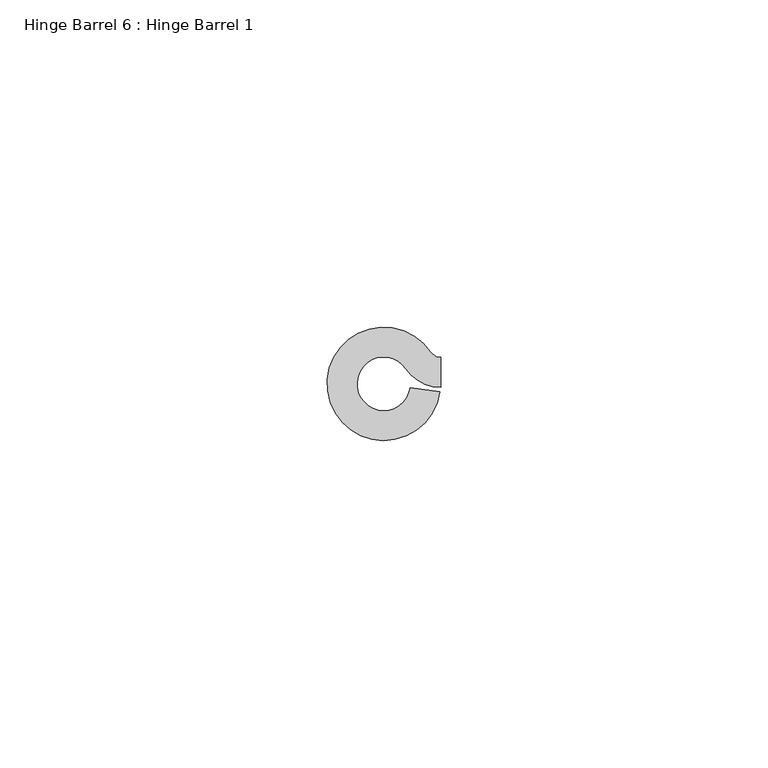
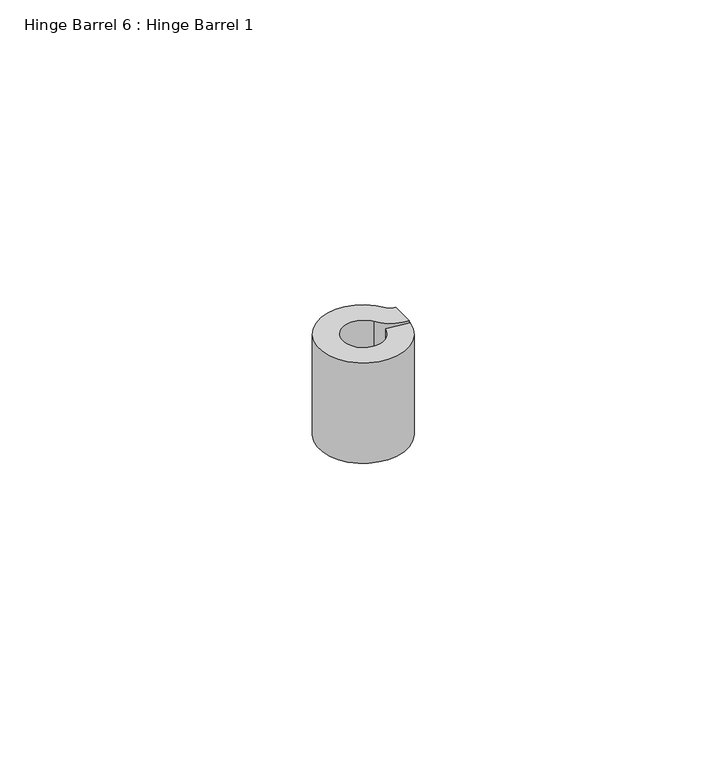
"""IFC4 building model written with IfcOpenShell, lengths in millimetres: proxy geometry, Hinge Barrel 6 : Hinge Barrel 1."""

import ifcopenshell
import ifcopenshell.guid

model = None  # the IFC model being written
_history = None  # IfcOwnerHistory: only IFC2X3 demands one
_inside = {}  # id of a spatial element -> (the spatial element, [elements in it])
_under = {}  # id of a project, library or spatial element -> (it, [spatial elements below it])
_declared = {}  # id of a project -> (the project, [libraries it declares])
_typed = {}  # id of a type object -> (the type object, [elements of that type])
_made_of = {}  # id of a material, layer set ... -> (it, [elements and type objects made of it])


def new_model(schema):
    """Start an empty IFC model of exactly this schema.

    Asked for "IFC4X3", IfcOpenShell would pick the latest addendum, in which some entities
    have other attributes; the version numbers below select the first issue.
    IFC2X3 requires an IfcOwnerHistory on every rooted entity: one is made here for all.
    """
    global model, _history
    if schema == "IFC4X3":
        model = ifcopenshell.file(schema_version=(4, 3, 0, 0))
    else:
        model = ifcopenshell.file(schema=schema)
    _inside.clear()
    _under.clear()
    _declared.clear()
    _typed.clear()
    _made_of.clear()
    _history = None
    if model.schema == "IFC2X3":
        org = make("IfcOrganization", Name="unknown")
        user = make(
            "IfcPersonAndOrganization",
            ThePerson=make("IfcPerson", FamilyName="unknown"),
            TheOrganization=org,
        )
        app = make(
            "IfcApplication",
            ApplicationDeveloper=org,
            Version="unknown",
            ApplicationFullName="unknown",
            ApplicationIdentifier="unknown",
        )
        _history = make(
            "IfcOwnerHistory",
            OwningUser=user,
            OwningApplication=app,
            ChangeAction="ADDED",
            CreationDate=0,
        )
    return model


def make(cls, **values):
    """One entity of the class cls with the attributes given. An attribute that is None is left unset."""
    return model.create_entity(
        cls, **{name: value for name, value in values.items() if value is not None}
    )


def rooted(cls, **values):
    """An entity with a GlobalId (a new one), such as an element, a storey or a relation."""
    return make(cls, GlobalId=ifcopenshell.guid.new(), OwnerHistory=_history, **values)


def si_unit(unit_type, name, prefix=None):
    """IfcSIUnit, for example si_unit("LENGTHUNIT", "METRE", prefix="MILLI")."""
    return make("IfcSIUnit", UnitType=unit_type, Prefix=prefix, Name=name)


def assignment(units):
    """IfcUnitAssignment: the units of a project."""
    return None if units is None else make("IfcUnitAssignment", Units=units)


def point(xyz):
    """IfcCartesianPoint."""
    return None if xyz is None else make("IfcCartesianPoint", Coordinates=xyz)


def direction(xyz):
    """IfcDirection."""
    return None if xyz is None else make("IfcDirection", DirectionRatios=xyz)


def frame(location, z_axis=None, x_axis=None):
    """IfcAxis2Placement3D, a coordinate frame: its origin and axes. An axis left out is left unset."""
    return make(
        "IfcAxis2Placement3D",
        Location=point(location),
        Axis=direction(z_axis),
        RefDirection=direction(x_axis),
    )


def frame_2d(location, x_axis=None):
    """IfcAxis2Placement2D, a coordinate frame in the plane: its origin and x axis."""
    return make(
        "IfcAxis2Placement2D", Location=point(location), RefDirection=direction(x_axis)
    )


def origin():
    """The frame at (0, 0, 0) with its axes left unset."""
    return frame((0.0, 0.0, 0.0))


def place(relative_to, where):
    """IfcLocalPlacement: puts the frame where relative to a parent placement (None: the world)."""
    return make(
        "IfcLocalPlacement", PlacementRelTo=relative_to, RelativePlacement=where
    )


def context(
    kind, dimensions, precision=None, world=None, true_north=None, identifier=None
):
    """IfcGeometricRepresentationContext, for example the 3D "Model" context."""
    return make(
        "IfcGeometricRepresentationContext",
        ContextIdentifier=identifier,
        ContextType=kind,
        CoordinateSpaceDimension=dimensions,
        Precision=precision,
        WorldCoordinateSystem=world,
        TrueNorth=true_north,
    )


def project(units=None, contexts=None):
    """IfcProject with its units and contexts."""
    return rooted(
        "IfcProject",
        Name="project",
        RepresentationContexts=contexts,
        UnitsInContext=assignment(units),
    )


def spatial(cls, under=None, at=None, **own):
    """A site, building, storey or space (cls), placed at a placement, below another one or the project."""
    s = rooted(cls, ObjectPlacement=at, **own)
    if under is not None:
        _under.setdefault(under.id(), (under, []))[1].append(s)
    return s


def polyline(points):
    """IfcPolyline through the points."""
    return make("IfcPolyline", Points=[point(p) for p in points])


def circle_curve(where, radius):
    """IfcCircle in the frame where."""
    return make("IfcCircle", Position=where, Radius=radius)


def trimmed(basis, trim1, trim2, sense, master):
    """IfcTrimmedCurve: the piece of a basis curve between two trims."""
    return make(
        "IfcTrimmedCurve",
        BasisCurve=basis,
        Trim1=trim1,
        Trim2=trim2,
        SenseAgreement=sense,
        MasterRepresentation=master,
    )


def segment(curve, same_sense, transition):
    """IfcCompositeCurveSegment."""
    return make(
        "IfcCompositeCurveSegment",
        Transition=transition,
        SameSense=same_sense,
        ParentCurve=curve,
    )


def composite_curve(segments, self_intersect=None):
    """IfcCompositeCurve: segments joined end to end."""
    return make("IfcCompositeCurve", Segments=segments, SelfIntersect=self_intersect)


def outline(outer, holes=None, kind="AREA"):
    """IfcArbitraryClosedProfileDef: a profile drawn as a closed curve; with holes, ...WithVoids."""
    if holes is None:
        return make("IfcArbitraryClosedProfileDef", ProfileType=kind, OuterCurve=outer)
    return make(
        "IfcArbitraryProfileDefWithVoids",
        ProfileType=kind,
        OuterCurve=outer,
        InnerCurves=holes,
    )


def extrude(swept, where, along, depth):
    """IfcExtrudedAreaSolid: the profile swept, set in the frame where, extruded along a direction by depth."""
    return make(
        "IfcExtrudedAreaSolid",
        SweptArea=swept,
        Position=where,
        ExtrudedDirection=direction(along),
        Depth=depth,
    )


def shape(context_of_items, identifier, shape_type, items):
    """IfcShapeRepresentation: the items that make up one representation, for example the "Body"."""
    return make(
        "IfcShapeRepresentation",
        ContextOfItems=context_of_items,
        RepresentationIdentifier=identifier,
        RepresentationType=shape_type,
        Items=items,
    )


def source(mapping_origin, context_of_items, identifier, shape_type, items):
    """IfcRepresentationMap: a shape defined once, which mapped items show again and again."""
    return make(
        "IfcRepresentationMap",
        MappingOrigin=mapping_origin,
        MappedRepresentation=shape(context_of_items, identifier, shape_type, items),
    )


def transform(
    local_origin,
    x_axis=None,
    y_axis=None,
    z_axis=None,
    scale=None,
    scale2=None,
    scale3=None,
    uniform=True,
):
    """IfcCartesianTransformationOperator3D, or its non-uniform kind. x_axis, y_axis, z_axis: its Axis1, 2, 3."""
    if uniform:
        return make(
            "IfcCartesianTransformationOperator3D",
            Axis1=direction(x_axis),
            Axis2=direction(y_axis),
            LocalOrigin=point(local_origin),
            Scale=scale,
            Axis3=direction(z_axis),
        )
    return make(
        "IfcCartesianTransformationOperator3DnonUniform",
        Axis1=direction(x_axis),
        Axis2=direction(y_axis),
        LocalOrigin=point(local_origin),
        Scale=scale,
        Axis3=direction(z_axis),
        Scale2=scale2,
        Scale3=scale3,
    )


def mapped(mapping_source, mapping_target):
    """IfcMappedItem: shows the shape of a source again, moved by a transform."""
    return make(
        "IfcMappedItem", MappingSource=mapping_source, MappingTarget=mapping_target
    )


def made_of(thing, what):
    """Note that an element or type object is made of a material, layer set ...; save() writes the relation."""
    if what is not None:
        _made_of.setdefault(what.id(), (what, []))[1].append(thing)
    return thing


def element(
    cls,
    number,
    at=None,
    inside=None,
    cuts=None,
    type_object=None,
    material=None,
    context=None,
    identifier="Body",
    shape_type=None,
    held_by="IfcProductDefinitionShape",
    body=None,
    shapes=None,
    **own,
):
    """One element of the class cls, such as IfcWall. Its Tag is "e" and its number.

    at: its placement. inside: the storey or other place that contains it. cuts: it is an
    opening in that element (IfcRelVoidsElement). A single representation is given by context,
    identifier, shape_type and body (its items); several are given by shapes. held_by: the class
    of the entity that holds the representations. save() writes the other relations.
    """
    e = rooted(cls, Tag="e%d" % number, ObjectPlacement=at, **own)
    if body is not None:
        shapes = [shape(context, identifier, shape_type, body)]
    if shapes is not None:
        e.Representation = make(held_by, Representations=shapes)
    if inside is not None:
        _inside.setdefault(inside.id(), (inside, []))[1].append(e)
    if cuts is not None:
        rooted(
            "IfcRelVoidsElement", RelatingBuildingElement=cuts, RelatedOpeningElement=e
        )
    if type_object is not None:
        _typed.setdefault(type_object.id(), (type_object, []))[1].append(e)
    return made_of(e, material)


def aggregate(whole, parts):
    """IfcRelAggregates: a whole, such as a stair, and the parts it consists of."""
    return rooted("IfcRelAggregates", RelatingObject=whole, RelatedObjects=parts)


def save(model, path):
    """Write the relations noted so far, then the file.

    IfcRelAggregates (storeys below a building ...), IfcRelContainedInSpatialStructure (elements
    in a storey), IfcRelDefinesByType, IfcRelAssociatesMaterial and IfcRelDeclares: one each for
    every whole, place, type object, material and project.
    """
    for whole, parts in _under.values():
        aggregate(whole, parts)
    for where, things in _inside.values():
        rooted(
            "IfcRelContainedInSpatialStructure",
            RelatedElements=things,
            RelatingStructure=where,
        )
    for kind, things in _typed.values():
        rooted("IfcRelDefinesByType", RelatedObjects=things, RelatingType=kind)
    for what, things in _made_of.values():
        rooted("IfcRelAssociatesMaterial", RelatedObjects=things, RelatingMaterial=what)
    for by, libraries in _declared.values():
        rooted("IfcRelDeclares", RelatingContext=by, RelatedDefinitions=libraries)
    model.write(path)


def hinge_barrel_6_hinge_barrel_1_f6209b09(model_context):
    return source(origin(), model_context, "Body", "SweptSolid", [
        extrude(outline(composite_curve([segment(trimmed(circle_curve(frame_2d((587319.1320739, -531776.6049841)), 4.0894), [point((587322.5194669, -531774.3139665))], [point((587323.1821338, -531777.1708529))], True, "CARTESIAN"), True, "CONTINUOUS"), segment(polyline([(587323.1821338, -531777.1708529), (587327.7022899, -531777.8024028)]), True, "CONTINUOUS"), segment(trimmed(circle_curve(frame_2d((587319.1320739, -531776.6049841)), 8.6534625), [point((587327.7022899, -531777.8024028))], [point((587326.3000393, -531771.7570273))], False, "CARTESIAN"), True, "CONTINUOUS"), segment(trimmed(circle_curve(frame_2d((587327.8245257, -531770.7259615)), 1.8404226), [point((587326.3000393, -531771.7570273))], [point((587327.8245257, -531772.5663841))], True, "CARTESIAN"), True, "CONTINUOUS"), segment(polyline([(587327.8245257, -531772.5663841), (587327.8245257, -531777.1304466)]), True, "CONTINUOUS"), segment(trimmed(circle_curve(frame_2d((587327.8245257, -531770.7259615)), 6.4044851), [point((587327.8245257, -531777.1304466))], [point((587322.5194669, -531774.3139665))], False, "CARTESIAN"), True, "CONTINUOUS")], self_intersect=False)), frame((0.0, 0.0, 438.15), z_axis=(0.0, 0.0, 1.0), x_axis=(1.0, 0.0, 0.0)), (0.0, 0.0, 1.0), 20.8359375),
    ])


if __name__ == "__main__":
    model = new_model("IFC4")
    model_context = context("Model", 3, world=origin())
    ifc_project = project(units=[si_unit("LENGTHUNIT", "METRE", prefix="MILLI")], contexts=[model_context])
    site = spatial("IfcSite", under=ifc_project)
    building = spatial("IfcBuilding", under=site)
    placement = place(None, origin())
    hinge_barrel_6_hinge_barrel_1_shape = hinge_barrel_6_hinge_barrel_1_f6209b09(model_context)
    element("IfcBuildingElementProxy", 1, Name="Hinge Barrel 6 : Hinge Barrel 1", ObjectType="Hinge Barrel 6 : Hinge Barrel 1", at=placement, inside=building, context=model_context, shape_type="MappedRepresentation", body=[
        mapped(hinge_barrel_6_hinge_barrel_1_shape, transform((0.0, 0.0, 0.0), x_axis=(1.0, 0.0, 0.0), y_axis=(0.0, 1.0, 0.0), z_axis=(0.0, 0.0, 1.0))),
    ])
    save(model, "model.ifc")

# Revit data of these elements
# Element 1 (IfcBuildingElementProxy, "Hinge Barrel 6 : Hinge Barrel 1")
#   Materials on its faces: "6\"X6\" WELD-ON STL BUTT HINGE"
# Materials
#   "6\"X6\" WELD-ON STL BUTT HINGE": class "Metal", colour RGB 189 187 185, transparency 0, Description = "Carbon steel", Cost = 0
